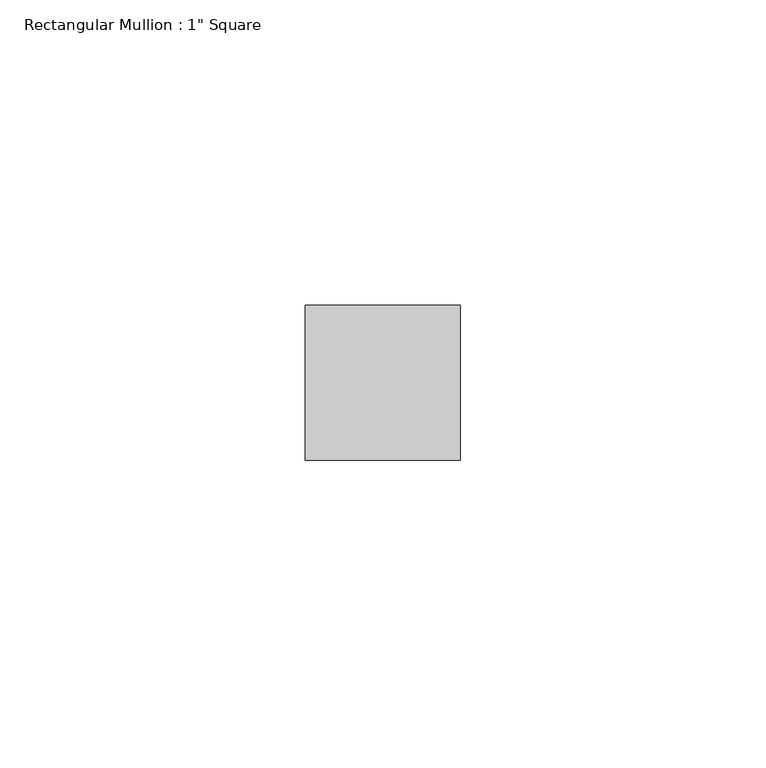
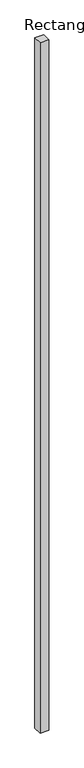
"""IFC4 building model written with IfcOpenShell, lengths in millimetres: member geometry."""

from ifc_helpers import new_model, si_unit, frame, origin, place, context, project, spatial, polyline, outline, extrude, source, transform, mapped, element, save


def member_da26c19c(model_context):
    return source(origin(), model_context, "Body", "SweptSolid", [
        extrude(outline(polyline([(0.0, 12.7), (0.0, -12.7), (-25.4, -12.7), (-25.4, 12.7), (0.0, 12.7)])), frame((0.0, 0.0, -2098.675), z_axis=(0.0, 0.0, 1.0), x_axis=(1.0, 0.0, 0.0)), (0.0, 0.0, 1.0), 2098.675),
    ])


if __name__ == "__main__":
    model = new_model("IFC4")
    model_context = context("Model", 3, world=origin())
    ifc_project = project(units=[si_unit("LENGTHUNIT", "METRE", prefix="MILLI")], contexts=[model_context])
    site = spatial("IfcSite", under=ifc_project)
    building = spatial("IfcBuilding", under=site)
    placement = place(None, origin())
    member_shape = member_da26c19c(model_context)
    element("IfcMember", 1, ObjectType="Rectangular Mullion : 1\" Square", at=placement, inside=building, context=model_context, shape_type="MappedRepresentation", body=[
        mapped(member_shape, transform((0.0, 0.0, 0.0), x_axis=(1.0, 0.0, 0.0), y_axis=(0.0, 1.0, 0.0), z_axis=(0.0, 0.0, 1.0))),
    ])
    save(model, "model.ifc")

# Revit data of these elements
# Type "Rectangular Mullion : 1\" Square"
#   built-in parameter 1007304 = 0.0833333 (stored number, unit not read)
#   built-in parameter 1007301 = 0.0416667 (stored number, unit not read)
#   built-in parameter 1007300 = 0.0416667 (stored number, unit not read)
# Element 1 (IfcMember, "Rectangular Mullion : 1\" Square")
#   Materials on its faces: "Metal - Aluminum"
# Materials
#   "Metal - Aluminum": class "Metal", colour RGB 247 247 247, transparency 0
